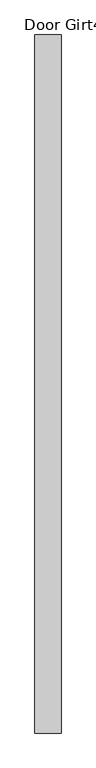
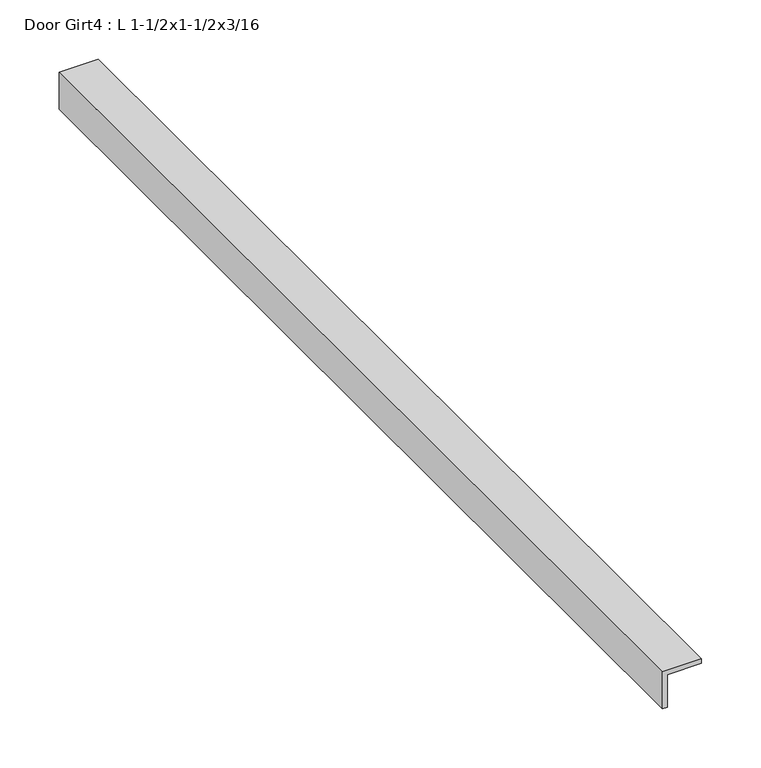
"""IFC4 building model written with IfcOpenShell, lengths in millimetres: proxy geometry, Door Girt4 : L 1-1/2x1-1/2x3/16."""

from ifc_helpers import new_model, si_unit, frame, origin, place, context, project, spatial, polyline, outline, extrude, source, transform, mapped, element, save


def door_girt4_l_1_1_2x1_1_2x3_16_372e9288(model_context):
    return source(origin(), model_context, "Body", "SweptSolid", [
        extrude(outline(polyline([(1625.6, 587403.9934739), (1625.6, 587365.8934739), (1587.5, 587365.8934739), (1587.5, 587370.6559739), (1620.8375, 587370.6559739), (1620.8375, 587403.9934739), (1625.6, 587403.9934739)])), frame((0.0, -536263.6038841, 0.0), z_axis=(0.0, 1.0, 0.0), x_axis=(0.0, 0.0, 1.0)), (0.0, 0.0, 1.0), 1017.5875),
    ])


if __name__ == "__main__":
    model = new_model("IFC4")
    model_context = context("Model", 3, world=origin())
    ifc_project = project(units=[si_unit("LENGTHUNIT", "METRE", prefix="MILLI")], contexts=[model_context])
    site = spatial("IfcSite", under=ifc_project)
    building = spatial("IfcBuilding", under=site)
    placement = place(None, origin())
    door_girt4_l_1_1_2x1_1_2x3_16_shape = door_girt4_l_1_1_2x1_1_2x3_16_372e9288(model_context)
    element("IfcBuildingElementProxy", 1, Name="Door Girt4 : L 1-1/2x1-1/2x3/16", ObjectType="Door Girt4 : L 1-1/2x1-1/2x3/16", at=placement, inside=building, context=model_context, shape_type="MappedRepresentation", body=[
        mapped(door_girt4_l_1_1_2x1_1_2x3_16_shape, transform((0.0, 0.0, 0.0), x_axis=(1.0, 0.0, 0.0), y_axis=(0.0, 1.0, 0.0), z_axis=(0.0, 0.0, 1.0))),
    ])
    save(model, "model.ifc")

# Revit data of these elements
# Element 1 (IfcBuildingElementProxy, "Door Girt4 : L 1-1/2x1-1/2x3/16")
#   Materials on its faces: "1-1/2\"X1-1/2\" GALV. STL L"
# Materials
#   "1-1/2\"X1-1/2\" GALV. STL L": class "Generic", colour RGB 211 211 207, transparency 0, Cost = 0
